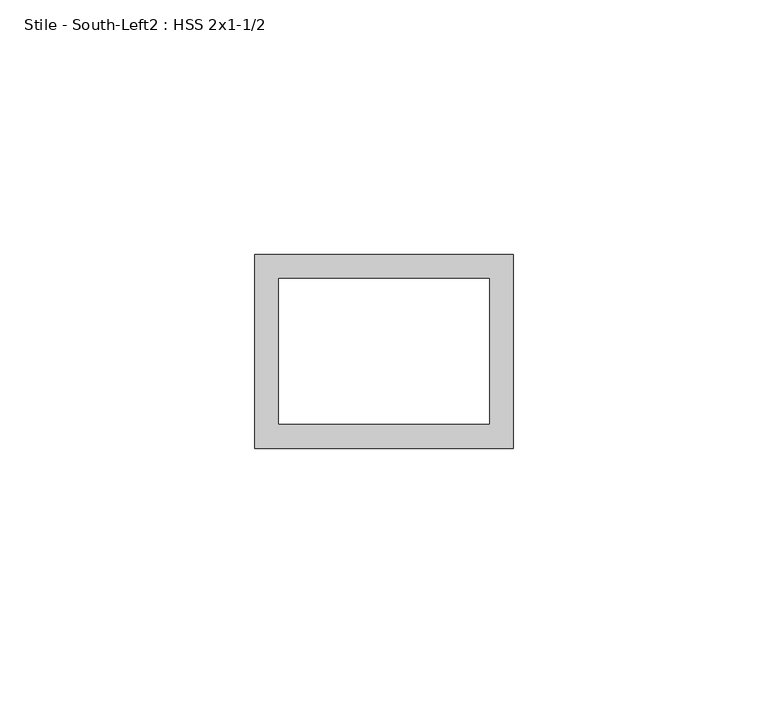
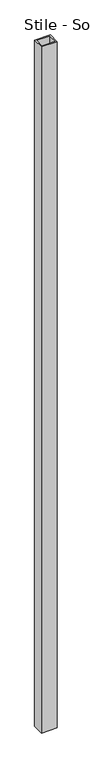
"""IFC4 building model written with IfcOpenShell, lengths in millimetres: proxy geometry, Stile - South-Left2 : HSS 2x1-1/2."""

from ifc_helpers import new_model, si_unit, frame, origin, place, context, project, spatial, polyline, outline, extrude, source, transform, mapped, element, save


def stile_south_left2_hss_2x1_1_2_374c26f2(model_context):
    return source(origin(), model_context, "Body", "SweptSolid", [
        extrude(outline(polyline([(587365.8934739, -532883.8163841), (587416.6934739, -532883.8163841), (587416.6934739, -532921.9163841), (587365.8934739, -532921.9163841), (587365.8934739, -532883.8163841)]), holes=[polyline([(587370.6559739, -532888.5788841), (587370.6559739, -532917.1538841), (587411.9309739, -532917.1538841), (587411.9309739, -532888.5788841), (587370.6559739, -532888.5788841)])]), frame((0.0, 0.0, 50.8), z_axis=(0.0, 0.0, 1.0), x_axis=(1.0, 0.0, 0.0)), (0.0, 0.0, 1.0), 2349.5),
    ])


if __name__ == "__main__":
    model = new_model("IFC4")
    model_context = context("Model", 3, world=origin())
    ifc_project = project(units=[si_unit("LENGTHUNIT", "METRE", prefix="MILLI")], contexts=[model_context])
    site = spatial("IfcSite", under=ifc_project)
    building = spatial("IfcBuilding", under=site)
    placement = place(None, origin())
    stile_south_left2_hss_2x1_1_2_shape = stile_south_left2_hss_2x1_1_2_374c26f2(model_context)
    element("IfcBuildingElementProxy", 1, Name="Stile - South-Left2 : HSS 2x1-1/2", ObjectType="Stile - South-Left2 : HSS 2x1-1/2", at=placement, inside=building, context=model_context, shape_type="MappedRepresentation", body=[
        mapped(stile_south_left2_hss_2x1_1_2_shape, transform((0.0, 0.0, 0.0), x_axis=(1.0, 0.0, 0.0), y_axis=(0.0, 1.0, 0.0), z_axis=(0.0, 0.0, 1.0))),
    ])
    save(model, "model.ifc")

# Revit data of these elements
# Element 1 (IfcBuildingElementProxy, "Stile - South-Left2 : HSS 2x1-1/2")
#   Materials on its faces: "1-1/2\"X2\" GALV. STL HSS TUBING"
# Materials
#   "1-1/2\"X2\" GALV. STL HSS TUBING": class "Generic", colour RGB 211 211 207, transparency 0, Cost = 0
